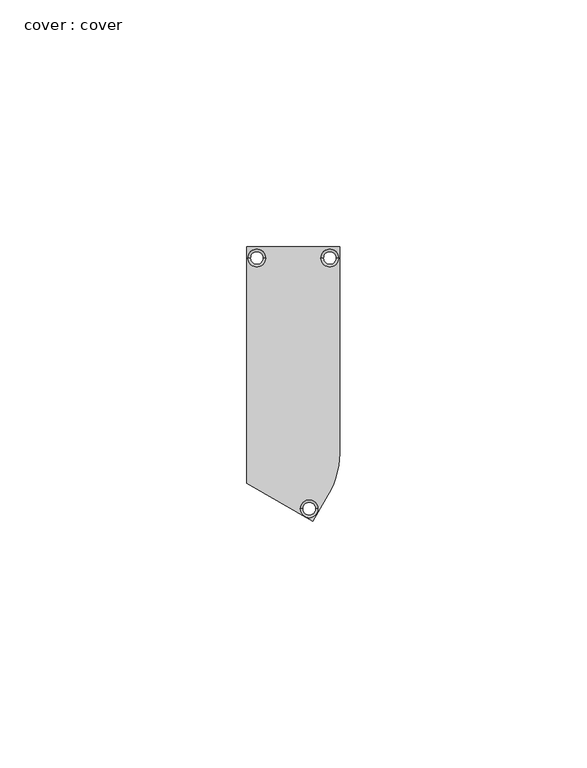
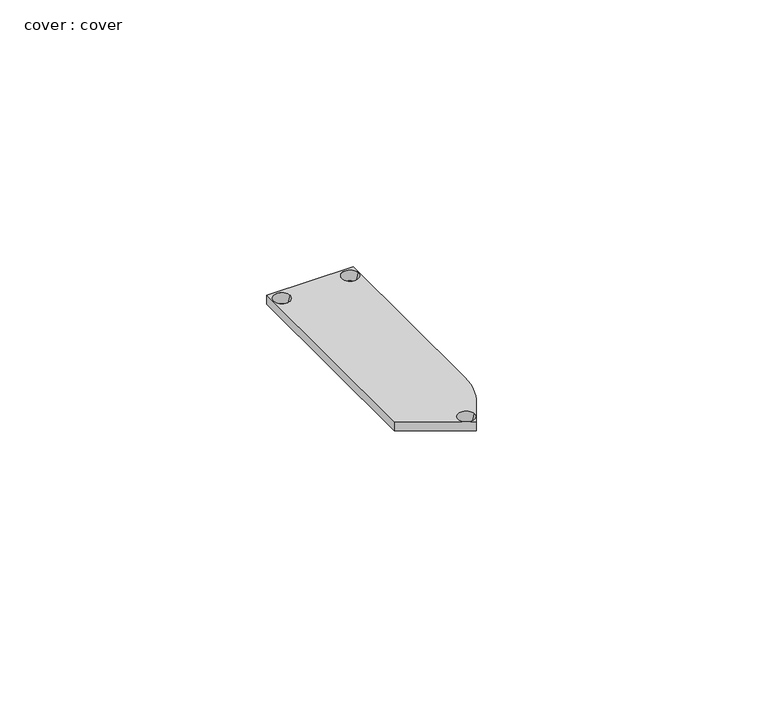
"""IFC4 building model written with IfcOpenShell, lengths in millimetres: proxy geometry, cover : cover."""

from ifc_helpers import new_model, si_unit, frame, origin, place, context, project, spatial, polyline, circle_curve, source, transform, mapped, element, save
from ifc_brep_helpers import plane_surface, revolved_surface, advanced_brep


def cover_cover_f3c25fb8(model_context):
    return source(origin(), model_context, "Body", "AdvancedBrep", [
        advanced_brep(
        [(4663.3311724, 3578.6670305, 2.0), (4663.3311724, 3530.8564939, 2.0), (4676.6686902, 3523.1530364, 2.0), (4680.3669524, 3529.5586705, 2.0), (4680.8851124, 3530.7118305, 2.0), (4681.3143724, 3531.9030905, 2.0), (4681.6547324, 3533.1222905, 2.0), (4681.9011124, 3534.3618105, 2.0), (4682.0560524, 3535.6191105, 2.0), (4682.1119324, 3536.8840305, 2.0), (4682.1119324, 3578.6670305, 2.0), (4667.1314224, 3576.4165905, 2.0), (4663.5314224, 3576.4165905, 2.0), (4681.9129524, 3576.4165905, 2.0), (4678.3129524, 3576.4165905, 2.0), (4677.7131366, 3525.6369105, 2.0), (4674.1587083, 3525.6369105, 2.0), (4663.3311724, 3578.6670305, 0.0), (4682.1119324, 3578.6670305, 0.0), (4682.1119324, 3536.8840305, 0.0), (4682.0560524, 3535.6191105, 0.0), (4681.9011124, 3534.3618105, 0.0), (4681.6547324, 3533.1222905, 0.0), (4681.3143724, 3531.9030905, 0.0), (4680.8851124, 3530.7118305, 0.0), (4680.3669524, 3529.5586705, 0.0), (4676.6686902, 3523.1530364, 0.0), (4663.3311724, 3530.8564939, 0.0), (4664.0314224, 3576.4165905, 0.0), (4666.6314224, 3576.4165905, 0.0), (4678.8129524, 3576.4165905, 0.0), (4681.4129524, 3576.4165905, 0.0), (4674.6206691, 3525.6369105, 0.0), (4677.2511758, 3525.6369105, 0.0)],
        [
            (0, 1),
            (1, 2),
            (2, 3),
            (3, 4),
            (4, 5),
            (5, 6),
            (6, 7),
            (7, 8),
            (8, 9),
            (9, 10),
            (10, 0),
            (11, 12, circle_curve(frame((4665.3314224, 3576.4165905, 2.0), z_axis=(0.0, 0.0, -1.0), x_axis=(-1.0, 0.0, 0.0)), 1.8)),
            (12, 11, circle_curve(frame((4665.3314224, 3576.4165905, 2.0), z_axis=(0.0, 0.0, -1.0), x_axis=(1.0, 0.0, 0.0)), 1.8)),
            (13, 14, circle_curve(frame((4680.1129524, 3576.4165905, 2.0), z_axis=(0.0, 0.0, -1.0), x_axis=(-1.0, 0.0, 0.0)), 1.8)),
            (14, 13, circle_curve(frame((4680.1129524, 3576.4165905, 2.0), z_axis=(0.0, 0.0, -1.0), x_axis=(1.0, 0.0, 0.0)), 1.8)),
            (15, 16, circle_curve(frame((4675.9359224, 3525.6369105, 2.0), z_axis=(0.0, 0.0, -1.0), x_axis=(-1.0, 0.0, 0.0)), 1.7772142)),
            (16, 15, circle_curve(frame((4675.9359224, 3525.6369105, 2.0), z_axis=(0.0, 0.0, -1.0), x_axis=(1.0, 0.0, 0.0)), 1.7772142)),
            (17, 18),
            (18, 19),
            (19, 20),
            (20, 21),
            (21, 22),
            (22, 23),
            (23, 24),
            (24, 25),
            (25, 26),
            (26, 27),
            (27, 17),
            (28, 29, circle_curve(frame((4665.3314224, 3576.4165905, 0.0), z_axis=(0.0, 0.0, 1.0), x_axis=(-1.0, 0.0, 0.0)), 1.3)),
            (29, 28, circle_curve(frame((4665.3314224, 3576.4165905, 0.0), z_axis=(0.0, 0.0, 1.0), x_axis=(1.0, 0.0, 0.0)), 1.3)),
            (30, 31, circle_curve(frame((4680.1129524, 3576.4165905, 0.0), z_axis=(0.0, 0.0, 1.0), x_axis=(-1.0, 0.0, 0.0)), 1.3)),
            (31, 30, circle_curve(frame((4680.1129524, 3576.4165905, 0.0), z_axis=(0.0, 0.0, 1.0), x_axis=(1.0, 0.0, 0.0)), 1.3)),
            (32, 33, circle_curve(frame((4675.9359224, 3525.6369105, 0.0), z_axis=(0.0, 0.0, 1.0), x_axis=(-1.0, 0.0, 0.0)), 1.3152534)),
            (33, 32, circle_curve(frame((4675.9359224, 3525.6369105, 0.0), z_axis=(0.0, 0.0, 1.0), x_axis=(1.0, 0.0, 0.0)), 1.3152534)),
            (0, 17),
            (27, 1),
            (26, 2),
            (25, 3),
            (9, 19),
            (18, 10),
            (24, 4),
            (23, 5),
            (22, 6),
            (21, 7),
            (20, 8),
            (28, 12),
            (11, 29),
            (30, 14),
            (13, 31),
            (32, 16),
            (15, 33),
        ],
        [
            plane_surface(frame((4663.3311724, 3531.8548305, 2.0), z_axis=(0.0, 0.0, 1.0), x_axis=(0.0, -1.0, 0.0))),
            plane_surface(frame((4663.3311724, 3531.8548305, 0.0), z_axis=(0.0, 0.0, -1.0), x_axis=(0.0, 1.0, 0.0))),
            plane_surface(frame((4663.3311724, 3578.6670305, 2.0), z_axis=(-1.0, 0.0, 0.0), x_axis=(0.0, 0.0, -1.0))),
            plane_surface(frame((4663.3311724, 3530.8564939, 2.0), z_axis=(-0.5001479267947538, -0.8659399813629751, 0.0), x_axis=(0.0, 0.0, -1.0))),
            plane_surface(frame((4676.6686902, 3523.1530364, 2.0), z_axis=(0.8660272939548952, -0.49999672611444335, 0.0), x_axis=(0.0, 0.0, -1.0))),
            plane_surface(frame((4682.1119324, 3536.8840305, 2.0), z_axis=(1.0, 0.0, 0.0), x_axis=(0.0, 0.0, -1.0))),
            plane_surface(frame((4680.3669524, 3529.5586705, 2.0), z_axis=(0.91214692510674, -0.40986337603928397, 0.0), x_axis=(0.0, 0.0, -1.0))),
            plane_surface(frame((4680.8851124, 3530.7118305, 2.0), z_axis=(0.9407850831608502, -0.3390035800725891, 0.0), x_axis=(0.0, 0.0, -1.0))),
            plane_surface(frame((4681.3143724, 3531.9030905, 2.0), z_axis=(0.9631721335643817, -0.26888555395379093, 0.0), x_axis=(0.0, 0.0, -1.0))),
            plane_surface(frame((4681.6547324, 3533.1222905, 2.0), z_axis=(0.9808118970912181, -0.19495646315094542, 0.0), x_axis=(0.0, 0.0, -1.0))),
            plane_surface(frame((4681.9011124, 3534.3618105, 2.0), z_axis=(0.9924922999614717, -0.12230713191465294, 0.0), x_axis=(0.0, 0.0, -1.0))),
            plane_surface(frame((4682.0560524, 3535.6191105, 2.0), z_axis=(0.9990256352193916, -0.04413366260000536, 0.0), x_axis=(0.0, 0.0, -1.0))),
            plane_surface(frame((4682.1119324, 3578.6670305, 2.0), z_axis=(0.0, 1.0, 0.0), x_axis=(0.0, 0.0, -1.0))),
            revolved_surface(polyline([(4663.5314224, 3576.4165905, 2.0), (4664.0314224, 3576.4165905, 0.0)]), (4665.3314224, 3576.4165905, -5.2), (0.0, 0.0, 1.0)),
            revolved_surface(polyline([(4678.3129524, 3576.4165905, 2.0), (4678.8129524, 3576.4165905, 0.0)]), (4680.1129524, 3576.4165905, -5.2), (0.0, 0.0, 1.0)),
            revolved_surface(polyline([(4674.1587083, 3525.6369105, 2.0), (4674.620669086516, 3525.6369105, 0.0)]), (4675.9359224, 3525.6369105, -5.6942206), (0.0, 0.0, 1.0)),
        ],
        [
            (0, [[1, 2, 3, 4, 5, 6, 7, 8, 9, 10, 11], [12, 13], [14, 15], [16, 17]]),
            (1, [[18, 19, 20, 21, 22, 23, 24, 25, 26, 27, 28], [29, 30], [31, 32], [33, 34]]),
            (2, [[-1, 35, -28, 36]]),
            (3, [[-2, -36, -27, 37]]),
            (4, [[-3, -37, -26, 38]]),
            (5, [[-10, 39, -19, 40]]),
            (6, [[-4, -38, -25, 41]]),
            (7, [[-5, -41, -24, 42]]),
            (8, [[-6, -42, -23, 43]]),
            (9, [[-7, -43, -22, 44]]),
            (10, [[-8, -44, -21, 45]]),
            (11, [[-9, -45, -20, -39]]),
            (12, [[-11, -40, -18, -35]]),
            (13, [[46, -12, 47, -29]]),
            (13, [[-46, -30, -47, -13]]),
            (14, [[48, -14, 49, -31]]),
            (14, [[-48, -32, -49, -15]]),
            (15, [[50, -16, 51, -33]]),
            (15, [[-50, -34, -51, -17]]),
        ],
    ),
    ])


if __name__ == "__main__":
    model = new_model("IFC4")
    model_context = context("Model", 3, world=origin())
    ifc_project = project(units=[si_unit("LENGTHUNIT", "METRE", prefix="MILLI")], contexts=[model_context])
    site = spatial("IfcSite", under=ifc_project)
    building = spatial("IfcBuilding", under=site)
    placement = place(None, origin())
    cover_cover_shape = cover_cover_f3c25fb8(model_context)
    element("IfcBuildingElementProxy", 1, Name="cover : cover", ObjectType="cover : cover", at=placement, inside=building, context=model_context, shape_type="MappedRepresentation", body=[
        mapped(cover_cover_shape, transform((0.0, 0.0, 0.0), x_axis=(1.0, 0.0, 0.0), y_axis=(0.0, 1.0, 0.0), z_axis=(0.0, 0.0, 1.0))),
    ])
    save(model, "model.ifc")
